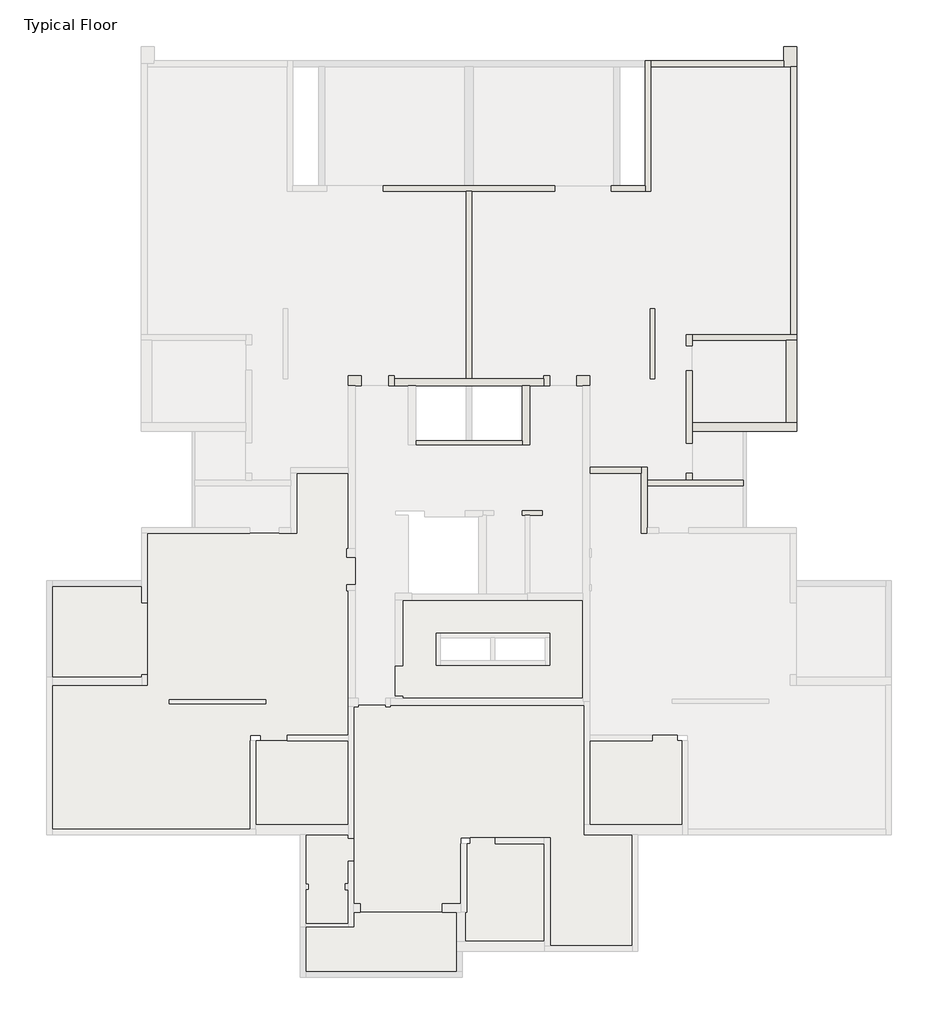
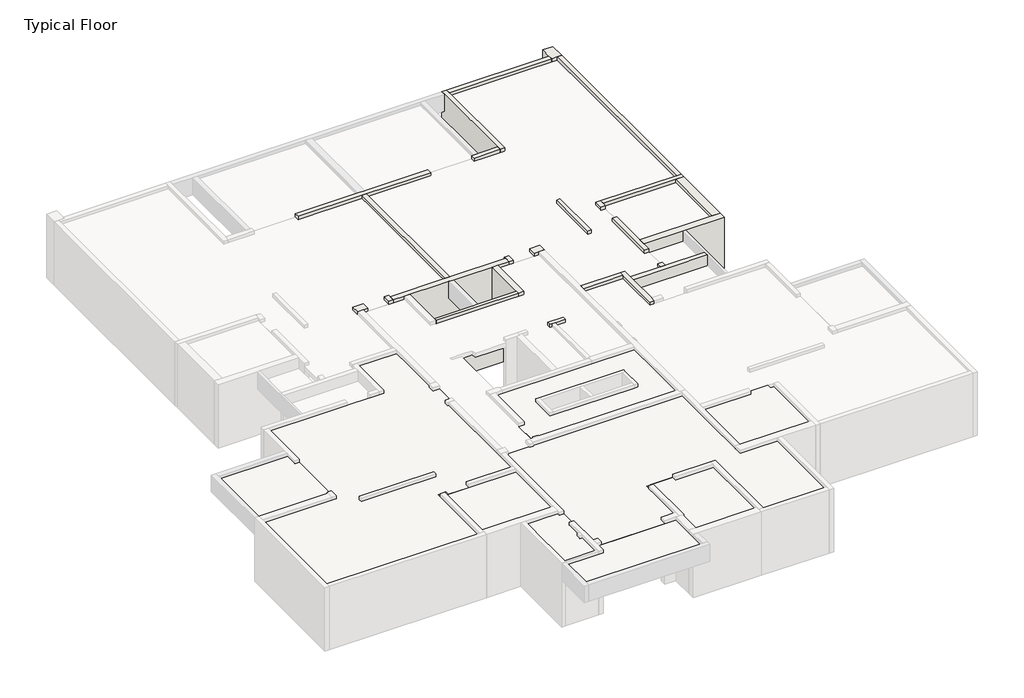
# One storey, part 3 of 4: 25 walls, 9 slabs.
"""IFC4 building model written with IfcOpenShell, lengths in millimetres."""

from ifc_helpers import new_model, si_unit, frame, origin, place, context, project, spatial, polyline, outline, extrude, faceted_brep, element, save

model = new_model("IFC4")

# Units and contexts
model_context = context("Model", 3, world=origin())
ifc_project = project(units=[si_unit("LENGTHUNIT", "METRE", prefix="MILLI")], contexts=[model_context])

# Site, building, storey
site = spatial("IfcSite", under=ifc_project)
building = spatial("IfcBuilding", under=site)
storey = spatial("IfcBuildingStorey", under=building, Name="Typical Floor", Elevation=3160.0)

# Slabs
placement = place(None, origin())
element("IfcSlab", 1, ObjectType="D=20", at=placement, inside=storey, context=model_context, shape_type="Brep", body=[
    faceted_brep([(353.6524939, -7625.251138, 2810.0), (353.6524939, -10519.1739201, 2810.0), (-2825.7294994, -10519.1739201, 2810.0), (-2825.7294994, -7625.251138, 2810.0), (-2665.7294994, -7625.251138, 2810.0), (-1746.3475061, -7625.251138, 2810.0), (353.6524939, -7625.251138, 3010.0), (-1746.3475061, -7625.251138, 3010.0), (-2665.7294994, -7625.251138, 3010.0), (-2825.7294994, -7625.251138, 3010.0), (-2825.7294994, -10519.1739201, 3010.0), (353.6524939, -10519.1739201, 3010.0)], [[[0, 1, 2, 3, 4, 5]], [[6, 7, 8, 9, 10, 11]], [[1, 0, 6, 11]], [[2, 1, 11, 10]], [[3, 2, 10, 9]], [[0, 5, 4, 3, 9, 8, 7, 6]]]),
])
element("IfcSlab", 2, ObjectType="D=20", at=placement, inside=storey, context=model_context, shape_type="SweptSolid", body=[
    extrude(outline(polyline([(353.6524939, -12752.8550877), (353.6524939, -13927.6329213), (-1104.0660909, -13927.6329213), (-1104.0660909, -12752.8550877), (-1004.0660909, -12752.8550877), (-1004.0660909, -12552.855147), (-1104.0660316, -12552.855147), (-1104.0660316, -10869.1739201), (353.6524939, -10869.1739201), (353.6524939, -10989.1739201), (553.6524939, -10989.1739201), (553.6524939, -11774.1739201), (353.6524939, -11774.1739201), (353.6524939, -12552.8550877), (253.6524939, -12552.8550877), (253.6524939, -12752.8550877), (353.6524939, -12752.8550877)])), frame((0.0, 0.0, 2810.0), z_axis=(0.0, 0.0, 1.0), x_axis=(1.0, 0.0, 0.0)), (0.0, 0.0, 1.0), 200.0),
])
element("IfcSlab", 3, ObjectType="D=20", at=placement, inside=storey, context=model_context, shape_type="Brep", body=[
    faceted_brep([(769.5270528, -13247.809147, 2810.0), (553.6524939, -13247.809147, 2810.0), (553.6524939, -11774.1739201, 2810.0), (553.6524939, -10989.1739201, 2810.0), (553.6524939, -6450.4733638, 2810.0), (703.0584279, -6450.4733638, 2810.0), (703.0584279, -6400.4733638, 2810.0), (1644.8990117, -6400.4733638, 2810.0), (1644.8990117, -6450.4733638, 2810.0), (1804.8990117, -6450.4733638, 2810.0), (1804.8990117, -6400.4733638, 2810.0), (8489.2361919, -6400.4733638, 2810.0), (8489.2361919, -10519.1739201, 2810.0), (8489.2361919, -10869.1739201, 2810.0), (10148.1730809, -10869.1739201, 2810.0), (10148.1730809, -14684.0133443, 2810.0), (7323.2436151, -14684.0133443, 2810.0), (7323.2436151, -10973.6256761, 2810.0), (7123.2436151, -10973.6256761, 2810.0), (5423.2436151, -10973.6256761, 2810.0), (4561.3412033, -10973.6256761, 2810.0), (4241.3412033, -10973.6256761, 2810.0), (4241.3412033, -11173.6256761, 2810.0), (4241.3412033, -13247.809147, 2810.0), (3603.9523756, -13247.809147, 2810.0), (3603.9523756, -13527.809147, 2810.0), (769.5270528, -13527.809147, 2810.0), (553.6524939, -13247.809147, 3010.0), (769.5270528, -13247.809147, 3010.0), (769.5270528, -13527.809147, 3010.0), (3603.9523756, -13527.809147, 3010.0), (3603.9523756, -13247.809147, 3010.0), (4241.3412033, -13247.809147, 3010.0), (4241.3412033, -11173.6256761, 3010.0), (4241.3412033, -10973.6256761, 3010.0), (4561.3412033, -10973.6256761, 3010.0), (5423.2436151, -10973.6256761, 3010.0), (7123.2436151, -10973.6256761, 3010.0), (7323.2436151, -10973.6256761, 3010.0), (7323.2436151, -14684.0133443, 3010.0), (10148.1730809, -14684.0133443, 3010.0), (10148.1730809, -10869.1739201, 3010.0), (8489.2361919, -10869.1739201, 3010.0), (8489.2361919, -10519.1739201, 3010.0), (8489.2361919, -6400.4733638, 3010.0), (1804.8990117, -6400.4733638, 3010.0), (1804.8990117, -6450.4733638, 3010.0), (1644.8990117, -6450.4733638, 3010.0), (1644.8990117, -6400.4733638, 3010.0), (703.0584279, -6400.4733638, 3010.0), (703.0584279, -6450.4733638, 3010.0), (553.6524939, -6450.4733638, 3010.0), (553.6524939, -10989.1739201, 3010.0), (553.6524939, -11774.1739201, 3010.0)], [[[0, 1, 2, 3, 4, 5, 6, 7, 8, 9, 10, 11, 12, 13, 14, 15, 16, 17, 18, 19, 20, 21, 22, 23, 24, 25, 26]], [[27, 28, 29, 30, 31, 32, 33, 34, 35, 36, 37, 38, 39, 40, 41, 42, 43, 44, 45, 46, 47, 48, 49, 50, 51, 52, 53]], [[1, 0, 28, 27]], [[4, 3, 2, 1, 27, 53, 52, 51]], [[5, 4, 51, 50]], [[6, 5, 50, 49]], [[7, 6, 49, 48]], [[8, 7, 48, 47]], [[9, 8, 47, 46]], [[10, 9, 46, 45]], [[11, 10, 45, 44]], [[11, 44, 43, 42, 13, 12]], [[14, 13, 42, 41]], [[15, 14, 41, 40]], [[16, 15, 40, 39]], [[17, 16, 39, 38]], [[17, 38, 37, 36, 35, 34, 21, 20, 19, 18]], [[21, 34, 33, 32, 23, 22]], [[24, 23, 32, 31]], [[25, 24, 31, 30]], [[26, 25, 30, 29]], [[0, 26, 29, 28]]]),
])
element("IfcSlab", 4, ObjectType="D=20", at=placement, inside=storey, context=model_context, shape_type="SweptSolid", body=[
    extrude(outline(polyline([(7123.2436151, -14534.1440447), (4393.8641143, -14534.1440447), (4393.8641143, -13527.809147), (4441.3412033, -13527.809147), (4441.3412033, -11173.6256761), (4561.3412033, -11173.6256761), (4561.3412033, -10973.6256761), (5423.2436151, -10973.6256761), (5423.2436151, -11173.6256761), (7123.2436151, -11173.6256761), (7123.2436151, -14534.1440447)])), frame((0.0, 0.0, 2810.0), z_axis=(0.0, 0.0, 1.0), x_axis=(1.0, 0.0, 0.0)), (0.0, 0.0, 1.0), 200.0),
])
element("IfcSlab", 5, ObjectType="D=20", at=placement, inside=storey, context=model_context, shape_type="SweptSolid", body=[
    extrude(outline(polyline([(11869.8374389, -7625.251138), (11869.8374389, -10519.1739201), (8689.2361919, -10519.1739201), (8689.2361919, -7625.251138), (10849.2361919, -7625.251138), (10849.2361919, -7425.251138), (11709.8374389, -7425.251138), (11709.8374389, -7625.251138), (11869.8374389, -7625.251138)])), frame((0.0, 0.0, 2810.0), z_axis=(0.0, 0.0, 1.0), x_axis=(1.0, 0.0, 0.0)), (0.0, 0.0, 1.0), 200.0),
])
element("IfcSlab", 6, ObjectType="D=20", at=placement, inside=storey, context=model_context, shape_type="Brep", body=[
    faceted_brep([(-9845.3223417, -10669.1739201, 2810.0), (-9845.3223417, -5707.6243159, 2810.0), (-6764.013165, -5707.6243159, 2810.0), (-6564.013165, -5707.6243159, 2810.0), (-6564.013165, -5351.6580536, 2810.0), (-6564.013165, -2868.5711301, 2810.0), (-6564.013165, -471.5347538, 2810.0), (-3044.013165, -471.5347538, 2810.0), (-2018.0126357, -471.5347538, 2810.0), (-1618.0126357, -471.5347538, 2810.0), (-1418.0126357, -471.5347538, 2810.0), (-1418.0126357, 1602.0583306, 2810.0), (353.0602083, 1602.0583306, 2810.0), (353.0602083, -998.8355577, 2810.0), (303.6507728, -998.8355577, 2810.0), (303.6507728, -1298.8355577, 2810.0), (603.0602083, -1298.8355577, 2810.0), (603.0602083, -2240.6761415, 2810.0), (303.6507728, -2240.6761415, 2810.0), (303.6507728, -2440.6761415, 2810.0), (353.6524939, -2440.6761415, 2810.0), (353.6524939, -6150.4733638, 2810.0), (353.6524939, -6450.4733638, 2810.0), (353.6524939, -7425.251138, 2810.0), (-1746.3475061, -7425.251138, 2810.0), (-1746.3475061, -7625.251138, 2810.0), (-2665.7294994, -7625.251138, 2810.0), (-2665.7294994, -7425.251138, 2810.0), (-3025.7294994, -7425.251138, 2810.0), (-3025.7294994, -7625.251138, 2810.0), (-3025.7294994, -10669.1739201, 2810.0), (-5822.171691, -6349.5529829, 2810.0), (-2483.2956212, -6349.5529829, 2810.0), (-2483.2956212, -6199.5529829, 2810.0), (-5822.171691, -6199.5529829, 2810.0), (-9845.3223417, -5707.6243159, 3010.0), (-9845.3223417, -10669.1739201, 3010.0), (-3025.7294994, -10669.1739201, 3010.0), (-3025.7294994, -7625.251138, 3010.0), (-3025.7294994, -7425.251138, 3010.0), (-2665.7294994, -7425.251138, 3010.0), (-2665.7294994, -7625.251138, 3010.0), (-1746.3475061, -7625.251138, 3010.0), (-1746.3475061, -7425.251138, 3010.0), (353.6524939, -7425.251138, 3010.0), (353.6524939, -6450.4733638, 3010.0), (353.6524939, -6150.4733638, 3010.0), (353.6524939, -2440.6761415, 3010.0), (303.6507728, -2440.6761415, 3010.0), (303.6507728, -2240.6761415, 3010.0), (603.0602083, -2240.6761415, 3010.0), (603.0602083, -1298.8355577, 3010.0), (303.6507728, -1298.8355577, 3010.0), (303.6507728, -998.8355577, 3010.0), (353.0602083, -998.8355577, 3010.0), (353.0602083, 1602.0583306, 3010.0), (-1418.0126357, 1602.0583306, 3010.0), (-1418.0126357, -471.5347538, 3010.0), (-1618.0126357, -471.5347538, 3010.0), (-2018.0126357, -471.5347538, 3010.0), (-3044.013165, -471.5347538, 3010.0), (-6564.013165, -471.5347538, 3010.0), (-6564.013165, -2868.5711301, 3010.0), (-6564.013165, -5351.6580536, 3010.0), (-6564.013165, -5707.6243159, 3010.0), (-6764.013165, -5707.6243159, 3010.0), (-2483.2956212, -6349.5529829, 3010.0), (-5822.171691, -6349.5529829, 3010.0), (-5822.171691, -6199.5529829, 3010.0), (-2483.2956212, -6199.5529829, 3010.0)], [[[0, 1, 2, 3, 4, 5, 6, 7, 8, 9, 10, 11, 12, 13, 14, 15, 16, 17, 18, 19, 20, 21, 22, 23, 24, 25, 26, 27, 28, 29, 30], [31, 32, 33, 34]], [[35, 36, 37, 38, 39, 40, 41, 42, 43, 44, 45, 46, 47, 48, 49, 50, 51, 52, 53, 54, 55, 56, 57, 58, 59, 60, 61, 62, 63, 64, 65], [66, 67, 68, 69]], [[1, 0, 36, 35]], [[1, 35, 65, 64, 3, 2]], [[3, 64, 63, 62, 61, 6, 5, 4]], [[6, 61, 60, 59, 58, 57, 10, 9, 8, 7]], [[11, 10, 57, 56]], [[12, 11, 56, 55]], [[13, 12, 55, 54]], [[14, 13, 54, 53]], [[15, 14, 53, 52]], [[16, 15, 52, 51]], [[17, 16, 51, 50]], [[18, 17, 50, 49]], [[19, 18, 49, 48]], [[20, 19, 48, 47]], [[20, 47, 46, 45, 44, 23, 22, 21]], [[28, 27, 40, 39]], [[28, 39, 38, 37, 30, 29]], [[0, 30, 37, 36]], [[32, 31, 67, 66]], [[34, 33, 69, 68]], [[33, 32, 66, 69]], [[31, 34, 68, 67]], [[24, 23, 44, 43]], [[25, 24, 43, 42]], [[26, 25, 42, 41]], [[27, 26, 41, 40]]]),
])
element("IfcSlab", 7, ObjectType="D=20", at=placement, inside=storey, context=model_context, shape_type="SweptSolid", body=[
    extrude(outline(polyline([(-9845.3223417, -2297.6508085), (-6764.013165, -2297.6508085), (-6764.013165, -2868.5711301), (-6564.013165, -2868.5711301), (-6564.013165, -5351.6580536), (-6764.013165, -5351.6580536), (-6764.013165, -5427.6243159), (-9845.3223417, -5427.6243159), (-9845.3223417, -2297.6508085)])), frame((0.0, 0.0, 2810.0), z_axis=(0.0, 0.0, 1.0), x_axis=(1.0, 0.0, 0.0)), (0.0, 0.0, 1.0), 200.0),
])
element("IfcSlab", 8, ObjectType="D=20", at=placement, inside=storey, context=model_context, shape_type="Brep", body=[
    faceted_brep([(353.6524939, -14027.6329213, 2810.0), (353.6524939, -14034.1739201, 2810.0), (553.6524939, -14034.1739201, 2810.0), (553.6524939, -13527.809147, 2810.0), (769.5270528, -13527.809147, 2810.0), (3603.9523756, -13527.809147, 2810.0), (4093.8641143, -13527.809147, 2810.0), (4093.8641143, -15583.8829405, 2810.0), (-1104.0660316, -15583.8829405, 2810.0), (-1104.0660316, -14027.6329213, 2810.0), (353.6524939, -14034.1739201, 3010.0), (353.6524939, -14027.6329213, 3010.0), (-1104.0660316, -14027.6329213, 3010.0), (-1104.0660316, -15583.8829405, 3010.0), (4093.8641143, -15583.8829405, 3010.0), (4093.8641143, -13527.809147, 3010.0), (3603.9523756, -13527.809147, 3010.0), (769.5270528, -13527.809147, 3010.0), (553.6524939, -13527.809147, 3010.0), (553.6524939, -14034.1739201, 3010.0)], [[[0, 1, 2, 3, 4, 5, 6, 7, 8, 9]], [[10, 11, 12, 13, 14, 15, 16, 17, 18, 19]], [[1, 0, 11, 10]], [[2, 1, 10, 19]], [[3, 2, 19, 18]], [[3, 18, 17, 16, 15, 6, 5, 4]], [[7, 6, 15, 14]], [[8, 7, 14, 13]], [[9, 8, 13, 12]], [[0, 9, 12, 11]]]),
])
element("IfcSlab", 9, ObjectType="D=20", at=placement, inside=storey, context=model_context, shape_type="Brep", body=[
    faceted_brep([(2237.3338395, -5031.1363023, 2810.0), (2237.3338395, -2776.1363023, 2810.0), (8439.2361919, -2776.1363023, 2810.0), (8439.2361919, -6150.4733638, 2810.0), (2237.3338395, -6150.4733638, 2810.0), (2237.3338395, -6084.0047389, 2810.0), (1987.3338395, -6084.0047389, 2810.0), (1987.3338395, -5031.1363023, 2810.0), (3385.5549057, -3915.4538564, 2810.0), (3385.5549057, -5009.2269053, 2810.0), (3535.5549057, -5009.2269053, 2810.0), (7154.2538596, -5009.2269053, 2810.0), (7304.2538596, -5009.2269053, 2810.0), (7304.2538596, -4065.4538564, 2810.0), (7304.2538596, -3915.4538564, 2810.0), (3535.5549057, -3915.4538564, 2810.0), (2237.3338395, -2776.1363023, 3010.0), (2237.3338395, -5031.1363023, 3010.0), (1987.3338395, -5031.1363023, 3010.0), (1987.3338395, -6084.0047389, 3010.0), (2237.3338395, -6084.0047389, 3010.0), (2237.3338395, -6150.4733638, 3010.0), (8439.2361919, -6150.4733638, 3010.0), (8439.2361919, -2776.1363023, 3010.0), (3385.5549057, -5009.2269053, 3010.0), (3385.5549057, -3915.4538564, 3010.0), (3535.5549057, -3915.4538564, 3010.0), (7304.2538596, -3915.4538564, 3010.0), (7304.2538596, -4065.4538564, 3010.0), (7304.2538596, -5009.2269053, 3010.0), (7154.2538596, -5009.2269053, 3010.0), (3535.5549057, -5009.2269053, 3010.0)], [[[0, 1, 2, 3, 4, 5, 6, 7], [8, 9, 10, 11, 12, 13, 14, 15]], [[16, 17, 18, 19, 20, 21, 22, 23], [24, 25, 26, 27, 28, 29, 30, 31]], [[1, 0, 17, 16]], [[2, 1, 16, 23]], [[3, 2, 23, 22]], [[4, 3, 22, 21]], [[5, 4, 21, 20]], [[6, 5, 20, 19]], [[7, 6, 19, 18]], [[0, 7, 18, 17]], [[29, 12, 11, 10, 9, 24, 31, 30]], [[12, 29, 28, 27, 14, 13]], [[14, 27, 26, 25, 8, 15]], [[9, 8, 25, 24]]]),
])

# Walls
element("IfcWall", 10, ObjectType="15", at=placement, inside=storey, context=model_context, shape_type="SweptSolid", body=[
    extrude(outline(polyline([(6359.8903055, 2582.4743311), (2684.2185243, 2582.4743311), (2684.2185243, 2732.4743311), (6359.8903055, 2732.4743311), (6359.8903055, 2582.4743311)])), frame((0.0, 0.0, 160.0), z_axis=(0.0, 0.0, 1.0), x_axis=(1.0, 0.0, 0.0)), (0.0, 0.0, 1.0), 3000.0),
])
element("IfcWall", 11, ObjectType="15", at=placement, inside=storey, context=model_context, shape_type="Brep", body=[
    faceted_brep([(7056.7750495, 306.3601755, 160.0), (6362.4114361, 306.3601755, 160.0), (6362.4114361, 306.3601755, 2810.0), (6362.4114361, 306.3601755, 3010.0), (6362.4114361, 306.3601755, 3160.0), (7056.7750495, 306.3601755, 3160.0), (7056.7750495, 306.3601755, 3010.0), (7056.7750495, 306.3601755, 2810.0), (7056.7750495, 156.3601755, 160.0), (7056.7750495, 156.3601755, 2810.0), (7056.7750495, 156.3601755, 3010.0), (7056.7750495, 156.3601755, 3160.0), (6609.8903055, 156.3601755, 3160.0), (6459.8903055, 156.3601755, 3160.0), (6362.4114361, 156.3601755, 3160.0), (6362.4114361, 156.3601755, 3010.0), (6362.4114361, 156.3601755, 2810.0), (6362.4114361, 156.3601755, 160.0), (6459.8903055, 156.3601755, 160.0), (6609.8903055, 156.3601755, 160.0)], [[[0, 1, 2, 3, 4, 5, 6, 7]], [[8, 9, 10, 11, 12, 13, 14, 15, 16, 17, 18, 19]], [[1, 0, 8, 19, 18, 17]], [[4, 3, 2, 1, 17, 16, 15, 14]], [[5, 4, 14, 13, 12, 11]], [[0, 7, 6, 5, 11, 10, 9, 8]]]),
])
element("IfcWall", 12, ObjectType="15", at=placement, inside=storey, context=model_context, shape_type="Brep", body=[
    faceted_brep([(10776.0680695, 7281.591066, 160.0), (10776.0680695, 4865.5631538, 160.0), (10776.0680695, 4865.5631538, 2810.0), (10776.0680695, 4865.5631538, 3010.0), (10776.0680695, 4865.5631538, 3160.0), (10776.0680695, 7281.591066, 3160.0), (10776.0680695, 7281.591066, 3010.0), (10776.0680695, 7281.591066, 2810.0), (10926.0680695, 7281.591066, 160.0), (10926.0680695, 7281.591066, 2810.0), (10926.0680695, 7281.591066, 3010.0), (10926.0680695, 7281.591066, 3160.0), (10926.0680695, 4865.5631538, 3160.0), (10926.0680695, 4865.5631538, 3010.0), (10926.0680695, 4865.5631538, 2810.0), (10926.0680695, 4865.5631538, 160.0)], [[[0, 1, 2, 3, 4, 5, 6, 7]], [[8, 9, 10, 11, 12, 13, 14, 15]], [[1, 0, 8, 15]], [[4, 3, 2, 1, 15, 14, 13, 12]], [[5, 4, 12, 11]], [[0, 7, 6, 5, 11, 10, 9, 8]]]),
])
element("IfcWall", 13, ObjectType="20", at=placement, inside=storey, context=model_context, shape_type="Brep", body=[
    faceted_brep([(10795.057825, 11324.9195447, 160.0), (10795.057825, 15624.6267847, 160.0), (10795.057825, 15824.6267847, 160.0), (10795.057825, 15824.6267847, 3160.0), (10795.057825, 15624.6267847, 3160.0), (10795.057825, 11324.9195447, 3160.0), (10795.057825, 11324.9195447, 3010.0), (10795.057825, 11324.9195447, 2810.0), (10595.057825, 11324.9195447, 160.0), (10595.057825, 11324.9195447, 3160.0), (10595.057825, 11524.9195447, 3160.0), (10595.057825, 15624.626844, 3160.0), (10595.057825, 15824.6267847, 3160.0), (10595.057825, 15824.6267847, 160.0), (10595.057825, 11524.9195447, 160.0)], [[[0, 1, 2, 3, 4, 5, 6, 7]], [[8, 9, 10, 11, 12, 13, 14]], [[2, 1, 0, 8, 14, 13]], [[5, 4, 3, 12, 11, 10, 9]], [[3, 2, 13, 12]], [[0, 7, 6, 5, 9, 8]]]),
])
element("IfcWall", 14, ObjectType="20", at=placement, inside=storey, context=model_context, shape_type="Brep", body=[
    faceted_brep([(10795.057825, 15624.6267847, 160.0), (15370.7330483, 15624.6267847, 160.0), (15370.7330483, 15624.6267847, 3160.0), (10795.057825, 15624.6267847, 3160.0), (10795.057825, 15624.6267847, 3010.0), (10795.057825, 15624.6267847, 2810.0), (10795.057825, 15824.6267847, 160.0), (10795.057825, 15824.6267847, 3160.0), (15370.7330483, 15824.6267847, 3160.0), (15370.7330483, 15824.6267847, 160.0)], [[[0, 1, 2, 3, 4, 5]], [[6, 7, 8, 9]], [[1, 0, 6, 9]], [[3, 2, 8, 7]], [[0, 5, 4, 3, 7, 6]], [[2, 1, 9, 8]]]),
])
element("IfcWall", 15, ObjectType="20", at=placement, inside=storey, context=model_context, shape_type="Brep", body=[
    faceted_brep([(15617.6160713, 15624.6267847, 160.0), (15617.6160713, 6387.8215778, 160.0), (15617.6160713, 6387.8215778, 2810.0), (15617.6160713, 6387.8215778, 3010.0), (15617.6160713, 6387.8215778, 3160.0), (15617.6160713, 15624.6267847, 3160.0), (15617.6160713, 15624.6267847, 3010.0), (15617.6160713, 15624.6267847, 2810.0), (15817.6160713, 15624.6267847, 160.0), (15817.6160713, 15624.6267847, 3160.0), (15817.6160713, 6387.8215778, 3160.0), (15817.6160713, 6387.8215778, 160.0)], [[[0, 1, 2, 3, 4, 5, 6, 7]], [[8, 9, 10, 11]], [[1, 0, 8, 11]], [[5, 4, 10, 9]], [[0, 7, 6, 5, 9, 8]], [[4, 3, 2, 1, 11, 10]]]),
])
element("IfcWall", 16, ObjectType="20", at=placement, inside=storey, context=model_context, shape_type="Brep", body=[
    faceted_brep([(15817.6160713, 6387.8215778, 160.0), (15617.6160713, 6387.8215778, 160.0), (12222.3603499, 6387.8215778, 160.0), (12222.3603499, 6387.8215778, 3160.0), (15617.6160713, 6387.8215778, 3160.0), (15817.6160713, 6387.8215778, 3160.0), (15817.6160713, 6187.8215778, 160.0), (15817.6160713, 6187.8215778, 3160.0), (15467.6160713, 6187.8215778, 3160.0), (12222.3603499, 6187.8215778, 3160.0), (12222.3603499, 6187.8215778, 160.0), (15467.6160713, 6187.8215778, 160.0)], [[[0, 1, 2, 3, 4, 5]], [[6, 7, 8, 9, 10, 11]], [[2, 1, 0, 6, 11, 10]], [[5, 4, 3, 9, 8, 7]], [[0, 5, 7, 6]], [[3, 2, 10, 9]]]),
])
element("IfcWall", 17, ObjectType="20", at=placement, inside=storey, context=model_context, shape_type="Brep", body=[
    faceted_brep([(12022.3603499, 5144.6693841, 160.0), (12022.3603499, 2644.6693841, 160.0), (12022.3603499, 2644.6693841, 2810.0), (12022.3603499, 2644.6693841, 3010.0), (12022.3603499, 2644.6693841, 3160.0), (12022.3603499, 5144.6693841, 3160.0), (12022.3603499, 5144.6693841, 3010.0), (12022.3603499, 5144.6693841, 2810.0), (12222.3603499, 5144.6693841, 160.0), (12222.3603499, 5144.6693841, 2810.0), (12222.3603499, 5144.6693841, 3010.0), (12222.3603499, 5144.6693841, 3160.0), (12222.3603499, 3348.3506111, 3160.0), (12222.3603499, 3048.3506111, 3160.0), (12222.3603499, 2644.6693841, 3160.0), (12222.3603499, 2644.6693841, 3010.0), (12222.3603499, 2644.6693841, 2810.0), (12222.3603499, 2644.6693841, 160.0), (12222.3603499, 3048.3506111, 160.0), (12222.3603499, 3348.3506111, 160.0)], [[[0, 1, 2, 3, 4, 5, 6, 7]], [[8, 9, 10, 11, 12, 13, 14, 15, 16, 17, 18, 19]], [[1, 0, 8, 19, 18, 17]], [[4, 3, 2, 1, 17, 16, 15, 14]], [[5, 4, 14, 13, 12, 11]], [[0, 7, 6, 5, 11, 10, 9, 8]]]),
])
element("IfcWall", 18, ObjectType="20", at=placement, inside=storey, context=model_context, shape_type="Brep", body=[
    faceted_brep([(4422.3514479, 11324.9195447, 160.0), (4422.3514479, 4865.5631538, 160.0), (4422.3514479, 4865.5631538, 2810.0), (4422.3514479, 4865.5631538, 3010.0), (4422.3514479, 4865.5631538, 3160.0), (4422.3514479, 11324.9195447, 3160.0), (4422.3514479, 11324.9195447, 3010.0), (4422.3514479, 11324.9195447, 2810.0), (4622.3514479, 11324.9195447, 160.0), (4622.3514479, 11324.9195447, 2810.0), (4622.3514479, 11324.9195447, 3010.0), (4622.3514479, 11324.9195447, 3160.0), (4622.3514479, 4865.5631538, 3160.0), (4622.3514479, 4865.5631538, 3010.0), (4622.3514479, 4865.5631538, 2810.0), (4622.3514479, 4865.5631538, 160.0)], [[[0, 1, 2, 3, 4, 5, 6, 7]], [[8, 9, 10, 11, 12, 13, 14, 15]], [[1, 0, 8, 15]], [[5, 4, 12, 11]], [[4, 3, 2, 1, 15, 14, 13, 12]], [[0, 7, 6, 5, 11, 10, 9, 8]]]),
])
element("IfcWall", 19, ObjectType="20", at=placement, inside=storey, context=model_context, shape_type="Brep", body=[
    faceted_brep([(1749.3507084, 4970.0149098, 160.0), (1749.3507084, 4615.5631538, 160.0), (1749.3507084, 4615.5631538, 2810.0), (1749.3507084, 4615.5631538, 3010.0), (1749.3507084, 4615.5631538, 3160.0), (1749.3507084, 4970.0149098, 3160.0), (1749.3507084, 4970.0149098, 3010.0), (1749.3507084, 4970.0149098, 2810.0), (1949.3507084, 4970.0149098, 160.0), (1949.3507084, 4970.0149098, 2810.0), (1949.3507084, 4970.0149098, 3010.0), (1949.3507084, 4970.0149098, 3160.0), (1949.3507084, 4865.5631538, 3160.0), (1949.3507084, 4615.5631538, 3160.0), (1949.3507084, 4615.5631538, 160.0), (1949.3507084, 4865.5631538, 160.0)], [[[0, 1, 2, 3, 4, 5, 6, 7]], [[8, 9, 10, 11, 12, 13, 14, 15]], [[1, 0, 8, 15, 14]], [[5, 4, 13, 12, 11]], [[0, 7, 6, 5, 11, 10, 9, 8]], [[4, 3, 2, 1, 14, 13]]]),
])
element("IfcWall", 20, ObjectType="20", at=placement, inside=storey, context=model_context, shape_type="Brep", body=[
    faceted_brep([(7104.8461452, 4970.0149098, 160.0), (7104.8461452, 4865.5631538, 160.0), (7104.8461452, 4615.5631538, 160.0), (7104.8461452, 4615.5631538, 3160.0), (7104.8461452, 4865.5631538, 3160.0), (7104.8461452, 4970.0149098, 3160.0), (7104.8461452, 4970.0149098, 3010.0), (7104.8461452, 4970.0149098, 2810.0), (7304.8461452, 4970.0149098, 160.0), (7304.8461452, 4970.0149098, 2810.0), (7304.8461452, 4970.0149098, 3010.0), (7304.8461452, 4970.0149098, 3160.0), (7304.8461452, 4615.5631538, 3160.0), (7304.8461452, 4615.5631538, 3010.0), (7304.8461452, 4615.5631538, 2810.0), (7304.8461452, 4615.5631538, 160.0)], [[[0, 1, 2, 3, 4, 5, 6, 7]], [[8, 9, 10, 11, 12, 13, 14, 15]], [[2, 1, 0, 8, 15]], [[5, 4, 3, 12, 11]], [[0, 7, 6, 5, 11, 10, 9, 8]], [[3, 2, 15, 14, 13, 12]]]),
])
element("IfcWall", 21, ObjectType="20", at=placement, inside=storey, context=model_context, shape_type="Brep", body=[
    faceted_brep([(13976.960118, 1364.6693841, 160.0), (12222.3603499, 1364.6693841, 160.0), (12022.3603499, 1364.6693841, 160.0), (10662.1205752, 1364.6693841, 160.0), (10662.1205752, 1364.6693841, 2810.0), (10662.1205752, 1364.6693841, 3010.0), (10662.1205752, 1364.6693841, 3160.0), (12022.3603499, 1364.6693841, 3160.0), (12222.3603499, 1364.6693841, 3160.0), (13976.960118, 1364.6693841, 3160.0), (13976.960118, 1364.6693841, 2660.0), (13976.960118, 1364.6693841, 2510.0), (13976.960118, 1164.6693841, 160.0), (13976.960118, 1164.6693841, 2510.0), (13976.960118, 1164.6693841, 2660.0), (13976.960118, 1164.6693841, 3160.0), (10662.1205752, 1164.6693841, 3160.0), (10662.1205752, 1164.6693841, 2660.0), (10662.1205752, 1164.6693841, 2510.0), (10662.1205752, 1164.6693841, 160.0)], [[[0, 1, 2, 3, 4, 5, 6, 7, 8, 9, 10, 11]], [[12, 13, 14, 15, 16, 17, 18, 19]], [[3, 2, 1, 0, 12, 19]], [[9, 8, 7, 6, 16, 15]], [[0, 11, 10, 9, 15, 14, 13, 12]], [[6, 5, 4, 3, 19, 18, 17, 16]]]),
])
element("IfcWall", 22, ObjectType="20", at=placement, inside=storey, context=model_context, shape_type="Brep", body=[
    faceted_brep([(10462.1205752, 1802.6523966, 160.0), (10462.1205752, 1602.6523966, 160.0), (10462.1205752, -471.5348131, 160.0), (10462.1205752, -471.5348131, 2810.0), (10462.1205752, -471.5348131, 3010.0), (10462.1205752, -471.5348131, 3160.0), (10462.1205752, 1602.6523966, 3160.0), (10462.1205752, 1802.6523966, 3160.0), (10662.1205752, 1802.6523966, 160.0), (10662.1205752, 1802.6523966, 2810.0), (10662.1205752, 1802.6523966, 3010.0), (10662.1205752, 1802.6523966, 3160.0), (10662.1205752, 1364.6693841, 3160.0), (10662.1205752, 1164.6693841, 3160.0), (10662.1205752, -271.5348131, 3160.0), (10662.1205752, -471.5348131, 3160.0), (10662.1205752, -471.5348131, 160.0), (10662.1205752, -271.5348131, 160.0), (10662.1205752, 1164.6693841, 160.0), (10662.1205752, 1364.6693841, 160.0)], [[[0, 1, 2, 3, 4, 5, 6, 7]], [[8, 9, 10, 11, 12, 13, 14, 15, 16, 17, 18, 19]], [[2, 1, 0, 8, 19, 18, 17, 16]], [[7, 6, 5, 15, 14, 13, 12, 11]], [[0, 7, 11, 10, 9, 8]], [[5, 4, 3, 2, 16, 15]]]),
])
element("IfcWall", 23, ObjectType="20", at=placement, inside=storey, context=model_context, shape_type="Brep", body=[
    faceted_brep([(8689.2361919, 1602.6523966, 160.0), (10462.1205752, 1602.6523966, 160.0), (10462.1205752, 1602.6523966, 2810.0), (10462.1205752, 1602.6523966, 3010.0), (10462.1205752, 1602.6523966, 3160.0), (8689.2361919, 1602.6523966, 3160.0), (8689.2361919, 1602.6523966, 3010.0), (8689.2361919, 1602.6523966, 2810.0), (8689.2361919, 1802.6523966, 160.0), (8689.2361919, 1802.6523966, 2810.0), (8689.2361919, 1802.6523966, 3010.0), (8689.2361919, 1802.6523966, 3160.0), (10462.1205752, 1802.6523966, 3160.0), (10462.1205752, 1802.6523966, 160.0)], [[[0, 1, 2, 3, 4, 5, 6, 7]], [[8, 9, 10, 11, 12, 13]], [[1, 0, 8, 13]], [[5, 4, 12, 11]], [[4, 3, 2, 1, 13, 12]], [[0, 7, 6, 5, 11, 10, 9, 8]]]),
])
element("IfcWall", 24, ObjectType="20", at=placement, inside=storey, context=model_context, shape_type="Brep", body=[
    faceted_brep([(10595.057825, 11524.9195447, 160.0), (9434.8198306, 11524.9195447, 160.0), (9434.8198306, 11524.9195447, 2810.0), (9434.8198306, 11524.9195447, 3010.0), (9434.8198306, 11524.9195447, 3160.0), (10595.057825, 11524.9195447, 3160.0), (10595.057825, 11324.9195447, 160.0), (10595.057825, 11324.9195447, 3160.0), (9434.8198306, 11324.9195447, 3160.0), (9434.8198306, 11324.9195447, 3010.0), (9434.8198306, 11324.9195447, 2810.0), (9434.8198306, 11324.9195447, 160.0)], [[[0, 1, 2, 3, 4, 5]], [[6, 7, 8, 9, 10, 11]], [[1, 0, 6, 11]], [[4, 3, 2, 1, 11, 10, 9, 8]], [[5, 4, 8, 7]], [[0, 5, 7, 6]]]),
])
element("IfcWall", 25, ObjectType="20", at=placement, inside=storey, context=model_context, shape_type="Brep", body=[
    faceted_brep([(7485.2622644, 11524.9195447, 160.0), (1568.9345892, 11524.9195447, 160.0), (1568.9345892, 11524.9195447, 2810.0), (1568.9345892, 11524.9195447, 3010.0), (1568.9345892, 11524.9195447, 3160.0), (7485.2622644, 11524.9195447, 3160.0), (7485.2622644, 11524.9195447, 3010.0), (7485.2622644, 11524.9195447, 2810.0), (7485.2622644, 11324.9195447, 160.0), (7485.2622644, 11324.9195447, 2810.0), (7485.2622644, 11324.9195447, 3010.0), (7485.2622644, 11324.9195447, 3160.0), (4622.3514479, 11324.9195447, 3160.0), (4422.3514479, 11324.9195447, 3160.0), (1568.9345892, 11324.9195447, 3160.0), (1568.9345892, 11324.9195447, 3010.0), (1568.9345892, 11324.9195447, 2810.0), (1568.9345892, 11324.9195447, 160.0), (4422.3514479, 11324.9195447, 160.0), (4622.3514479, 11324.9195447, 160.0)], [[[0, 1, 2, 3, 4, 5, 6, 7]], [[8, 9, 10, 11, 12, 13, 14, 15, 16, 17, 18, 19]], [[1, 0, 8, 19, 18, 17]], [[4, 3, 2, 1, 17, 16, 15, 14]], [[5, 4, 14, 13, 12, 11]], [[0, 7, 6, 5, 11, 10, 9, 8]]]),
])
element("IfcWall", 26, ObjectType="20", at=placement, inside=storey, context=model_context, shape_type="Brep", body=[
    faceted_brep([(12022.3603499, 6387.8215778, 160.0), (12022.3603499, 6007.8215778, 160.0), (12022.3603499, 6007.8215778, 2810.0), (12022.3603499, 6007.8215778, 3010.0), (12022.3603499, 6007.8215778, 3160.0), (12022.3603499, 6387.8215778, 3160.0), (12022.3603499, 6387.8215778, 3010.0), (12022.3603499, 6387.8215778, 2810.0), (12222.3603499, 6387.8215778, 160.0), (12222.3603499, 6387.8215778, 3160.0), (12222.3603499, 6187.8215778, 3160.0), (12222.3603499, 6007.8215778, 3160.0), (12222.3603499, 6007.8215778, 3010.0), (12222.3603499, 6007.8215778, 2810.0), (12222.3603499, 6007.8215778, 160.0), (12222.3603499, 6187.8215778, 160.0)], [[[0, 1, 2, 3, 4, 5, 6, 7]], [[8, 9, 10, 11, 12, 13, 14, 15]], [[1, 0, 8, 15, 14]], [[4, 3, 2, 1, 14, 13, 12, 11]], [[5, 4, 11, 10, 9]], [[0, 7, 6, 5, 9, 8]]]),
])
element("IfcWall", 27, ObjectType="20", at=placement, inside=storey, context=model_context, shape_type="Brep", body=[
    faceted_brep([(12022.3603499, 1602.6523966, 160.0), (12022.3603499, 1364.6693841, 160.0), (12022.3603499, 1364.6693841, 2810.0), (12022.3603499, 1364.6693841, 3010.0), (12022.3603499, 1364.6693841, 3160.0), (12022.3603499, 1602.6523966, 3160.0), (12022.3603499, 1602.6523966, 3010.0), (12022.3603499, 1602.6523966, 2810.0), (12222.3603499, 1602.6523966, 160.0), (12222.3603499, 1602.6523966, 2810.0), (12222.3603499, 1602.6523966, 3010.0), (12222.3603499, 1602.6523966, 3160.0), (12222.3603499, 1364.6693841, 3160.0), (12222.3603499, 1364.6693841, 160.0)], [[[0, 1, 2, 3, 4, 5, 6, 7]], [[8, 9, 10, 11, 12, 13]], [[1, 0, 8, 13]], [[5, 4, 12, 11]], [[0, 7, 6, 5, 11, 10, 9, 8]], [[4, 3, 2, 1, 13, 12]]]),
])
element("IfcWall", 28, ObjectType="25", at=placement, inside=storey, context=model_context, shape_type="Brep", body=[
    faceted_brep([(1949.3507084, 4615.5631538, 160.0), (2434.2185243, 4615.5631538, 160.0), (2684.2185243, 4615.5631538, 160.0), (6359.8903055, 4615.5631538, 160.0), (6609.8903055, 4615.5631538, 160.0), (7104.8461452, 4615.5631538, 160.0), (7104.8461452, 4615.5631538, 3160.0), (6609.8903055, 4615.5631538, 3160.0), (6359.8903055, 4615.5631538, 3160.0), (2684.2185243, 4615.5631538, 3160.0), (2434.2185243, 4615.5631538, 3160.0), (1949.3507084, 4615.5631538, 3160.0), (1949.3507084, 4865.5631538, 160.0), (1949.3507084, 4865.5631538, 2810.0), (1949.3507084, 4865.5631538, 3010.0), (1949.3507084, 4865.5631538, 3160.0), (4422.3514479, 4865.5631538, 3160.0), (4622.3514479, 4865.5631538, 3160.0), (7104.8461452, 4865.5631538, 3160.0), (7104.8461452, 4865.5631538, 3010.0), (7104.8461452, 4865.5631538, 2810.0), (7104.8461452, 4865.5631538, 160.0), (4622.3514479, 4865.5631538, 160.0), (4422.3514479, 4865.5631538, 160.0)], [[[0, 1, 2, 3, 4, 5, 6, 7, 8, 9, 10, 11]], [[12, 13, 14, 15, 16, 17, 18, 19, 20, 21, 22, 23]], [[5, 4, 3, 2, 1, 0, 12, 23, 22, 21]], [[11, 10, 9, 8, 7, 6, 18, 17, 16, 15]], [[0, 11, 15, 14, 13, 12]], [[6, 5, 21, 20, 19, 18]]]),
])
element("IfcWall", 29, ObjectType="25", at=placement, inside=storey, context=model_context, shape_type="Brep", body=[
    faceted_brep([(6609.8903055, 2582.4743311, 160.0), (6609.8903055, 4615.5631538, 160.0), (6609.8903055, 4615.5631538, 2810.0), (6609.8903055, 4615.5631538, 3010.0), (6609.8903055, 4615.5631538, 3160.0), (6609.8903055, 2582.4743311, 3160.0), (6609.8903055, 2582.4743311, 3010.0), (6609.8903055, 2582.4743311, 2810.0), (6359.8903055, 2582.4743311, 160.0), (6359.8903055, 2582.4743311, 3160.0), (6359.8903055, 2732.4743311, 3160.0), (6359.8903055, 4615.5631538, 3160.0), (6359.8903055, 4615.5631538, 160.0), (6359.8903055, 2732.4743311, 160.0)], [[[0, 1, 2, 3, 4, 5, 6, 7]], [[8, 9, 10, 11, 12, 13]], [[1, 0, 8, 13, 12]], [[5, 4, 11, 10, 9]], [[4, 3, 2, 1, 12, 11]], [[0, 7, 6, 5, 9, 8]]]),
])
element("IfcWall", 30, ObjectType="30", at=placement, inside=storey, context=model_context, shape_type="Brep", body=[
    faceted_brep([(12222.3603499, 3048.3506111, 160.0), (15817.6160713, 3048.3506111, 160.0), (15817.6160713, 3048.3506111, 3160.0), (12222.3603499, 3048.3506111, 3160.0), (12222.3603499, 3048.3506111, 2660.0), (12222.3603499, 3048.3506111, 2510.0), (12222.3603499, 3348.3506111, 160.0), (12222.3603499, 3348.3506111, 2810.0), (12222.3603499, 3348.3506111, 3010.0), (12222.3603499, 3348.3506111, 3160.0), (15467.6160713, 3348.3506111, 3160.0), (15817.6160713, 3348.3506111, 3160.0), (15817.6160713, 3348.3506111, 160.0), (15467.6160713, 3348.3506111, 160.0)], [[[0, 1, 2, 3, 4, 5]], [[6, 7, 8, 9, 10, 11, 12, 13]], [[1, 0, 6, 13, 12]], [[3, 2, 11, 10, 9]], [[0, 5, 4, 3, 9, 8, 7, 6]], [[2, 1, 12, 11]]]),
])
element("IfcWall", 31, ObjectType="35", at=placement, inside=storey, context=model_context, shape_type="Brep", body=[
    faceted_brep([(15467.6160713, 6187.8215778, 160.0), (15467.6160713, 3348.3506111, 160.0), (15467.6160713, 3348.3506111, 2810.0), (15467.6160713, 3348.3506111, 3010.0), (15467.6160713, 3348.3506111, 3160.0), (15467.6160713, 6187.8215778, 3160.0), (15817.6160713, 6187.8215778, 160.0), (15817.6160713, 6187.8215778, 3160.0), (15817.6160713, 3348.3506111, 3160.0), (15817.6160713, 3348.3506111, 160.0)], [[[0, 1, 2, 3, 4, 5]], [[6, 7, 8, 9]], [[1, 0, 6, 9]], [[5, 4, 8, 7]], [[0, 5, 7, 6]], [[4, 3, 2, 1, 9, 8]]]),
])
element("IfcWall", 32, ObjectType="45", at=placement, inside=storey, context=model_context, shape_type="Brep", body=[
    faceted_brep([(15370.7330483, 16318.9904575, 160.0), (15370.7330483, 15824.6267847, 160.0), (15370.7330483, 15624.6267847, 160.0), (15370.7330483, 15624.6267847, 3160.0), (15370.7330483, 15824.6267847, 3160.0), (15370.7330483, 16318.9904575, 3160.0), (15820.7330483, 16318.9904575, 160.0), (15820.7330483, 16318.9904575, 3160.0), (15820.7330483, 15624.6267847, 3160.0), (15820.7330483, 15624.6267847, 160.0), (15817.6160713, 15624.6267847, 160.0), (15617.6160713, 15624.6267847, 160.0), (15617.6160713, 15624.6267847, 3160.0), (15817.6160713, 15624.6267847, 3160.0)], [[[0, 1, 2, 3, 4, 5]], [[6, 7, 8, 9]], [[2, 1, 0, 6, 9, 10, 11]], [[5, 4, 3, 12, 13, 8, 7]], [[0, 5, 7, 6]], [[3, 2, 11, 10, 9, 8, 13, 12]]]),
])
element("IfcWall", 33, ObjectType="45", at=placement, inside=storey, context=model_context, shape_type="Brep", body=[
    faceted_brep([(8239.2361919, 4965.0149098, 160.0), (8239.2361919, 4613.0861241, 160.0), (8239.2361919, 4613.0861241, 2810.0), (8239.2361919, 4613.0861241, 3010.0), (8239.2361919, 4613.0861241, 3160.0), (8239.2361919, 4965.0149098, 3160.0), (8239.2361919, 4965.0149098, 3010.0), (8239.2361919, 4965.0149098, 2810.0), (8689.2361919, 4965.0149098, 160.0), (8689.2361919, 4965.0149098, 2810.0), (8689.2361919, 4965.0149098, 3010.0), (8689.2361919, 4965.0149098, 3160.0), (8689.2361919, 4613.0861241, 3160.0), (8689.2361919, 4613.0861241, 160.0), (8439.2361919, 4613.0861241, 160.0), (8439.2361919, 4613.0861241, 3160.0)], [[[0, 1, 2, 3, 4, 5, 6, 7]], [[8, 9, 10, 11, 12, 13]], [[1, 0, 8, 13, 14]], [[4, 3, 2, 1, 14, 13, 12, 15]], [[5, 4, 15, 12, 11]], [[0, 7, 6, 5, 11, 10, 9, 8]]]),
])
element("IfcWall", 34, ObjectType="45", at=placement, inside=storey, context=model_context, shape_type="Brep", body=[
    faceted_brep([(353.0602083, 4970.0149098, 160.0), (353.0602083, 4618.0861241, 160.0), (353.0602083, 4618.0861241, 3160.0), (353.0602083, 4970.0149098, 3160.0), (353.0602083, 4970.0149098, 3010.0), (353.0602083, 4970.0149098, 2810.0), (803.0602083, 4970.0149098, 160.0), (803.0602083, 4970.0149098, 2810.0), (803.0602083, 4970.0149098, 3010.0), (803.0602083, 4970.0149098, 3160.0), (803.0602083, 4618.0861241, 3160.0), (803.0602083, 4618.0861241, 3010.0), (803.0602083, 4618.0861241, 2810.0), (803.0602083, 4618.0861241, 160.0), (603.0602083, 4618.0861241, 160.0), (603.0602083, 4618.0861241, 3160.0)], [[[0, 1, 2, 3, 4, 5]], [[6, 7, 8, 9, 10, 11, 12, 13]], [[1, 0, 6, 13, 14]], [[2, 1, 14, 13, 12, 11, 10, 15]], [[3, 2, 15, 10, 9]], [[0, 5, 4, 3, 9, 8, 7, 6]]]),
])

save(model, "model.ifc")

# Revit data of these elements
# Type "D=20"
#   Function = 0
#   Layers, outside or top first: 20 cm "Concrete, Cast-in-Place - B30" (function 1)
# Type "15"
#   Layers, outside or top first: 15 cm "Concrete, Cast-in-Place - B30" (function 1)
# Type "20"
#   Layers, outside or top first: 20 cm "Concrete, Cast-in-Place - B30" (function 1)
# Type "25"
#   Layers, outside or top first: 25 cm "Concrete, Cast-in-Place - B30" (function 1)
# Type "30"
#   Layers, outside or top first: 30 cm "Concrete, Cast-in-Place - B30" (function 1)
# Type "35"
#   Layers, outside or top first: 35 cm "Concrete, Cast-in-Place - B30" (function 1)
# Type "45"
#   Layers, outside or top first: 45 cm "Concrete, Cast-in-Place - B30" (function 1)
# Element 1 (IfcSlab, "D=20")
#   Comments = ""
#   Mark = "S1"
#   SOFiSTiK_AMG_Comments = ""
#   Height Offset From Level = -15 cm
#   built-in parameter 1001954 = 1
#   SOFiSTiK_AMG_Scheduled = yes
#   SOFiSTiK_AMG_Adjusted = yes
#   Phase Created = New Construction
#   Materials on its faces: "Concrete, Cast-in-Place - B30"
# Element 2 (IfcSlab, "D=20")
#   Comments = ""
#   Mark = "S2"
#   SOFiSTiK_AMG_Comments = ""
#   Height Offset From Level = -15 cm
#   built-in parameter 1001954 = 1
#   SOFiSTiK_AMG_Scheduled = yes
#   SOFiSTiK_AMG_Adjusted = yes
#   Phase Created = New Construction
#   Materials on its faces: "Concrete, Cast-in-Place - B30"
# Element 3 (IfcSlab, "D=20")
#   Comments = ""
#   Mark = "S3"
#   SOFiSTiK_AMG_Comments = ""
#   Height Offset From Level = -15 cm
#   built-in parameter 1001954 = 1
#   SOFiSTiK_AMG_Scheduled = yes
#   SOFiSTiK_AMG_Adjusted = yes
#   Phase Created = New Construction
#   Materials on its faces: "Concrete, Cast-in-Place - B30"
# Element 4 (IfcSlab, "D=20")
#   Comments = ""
#   Mark = "S4"
#   SOFiSTiK_AMG_Comments = ""
#   Height Offset From Level = -15 cm
#   built-in parameter 1001954 = 1
#   SOFiSTiK_AMG_Scheduled = yes
#   SOFiSTiK_AMG_Adjusted = yes
#   Phase Created = New Construction
#   Materials on its faces: "Concrete, Cast-in-Place - B30"
# Element 5 (IfcSlab, "D=20")
#   Mark = "S5"
#   SOFiSTiK_AMG_Comments = ""
#   Height Offset From Level = -15 cm
#   built-in parameter 1001954 = 1
#   SOFiSTiK_AMG_Scheduled = yes
#   SOFiSTiK_AMG_Adjusted = yes
#   Phase Created = New Construction
#   Materials on its faces: "Concrete, Cast-in-Place - B30"
# Element 6 (IfcSlab, "D=20")
#   Mark = "S7"
#   SOFiSTiK_AMG_Comments = ""
#   built-in parameter 1001955 = 3.14159 (stored number, unit not read)
#   Height Offset From Level = -15 cm
#   built-in parameter 1001954 = 1
#   SOFiSTiK_AMG_Scheduled = yes
#   SOFiSTiK_AMG_Adjusted = yes
#   Phase Created = New Construction
#   Materials on its faces: "Concrete, Cast-in-Place - B30"
# Element 7 (IfcSlab, "D=20")
#   Mark = "S15"
#   SOFiSTiK_AMG_Comments = ""
#   built-in parameter 1001955 = 3.14159 (stored number, unit not read)
#   Height Offset From Level = -15 cm
#   built-in parameter 1001954 = 1
#   SOFiSTiK_AMG_Scheduled = yes
#   SOFiSTiK_AMG_Adjusted = yes
#   Phase Created = New Construction
#   Materials on its faces: "Concrete, Cast-in-Place - B30"
# Element 8 (IfcSlab, "D=20")
#   Mark = "S17"
#   SOFiSTiK_AMG_Comments = ""
#   Height Offset From Level = -15 cm
#   built-in parameter 1001954 = 1
#   SOFiSTiK_AMG_Scheduled = yes
#   SOFiSTiK_AMG_Adjusted = yes
#   Phase Created = New Construction
#   Materials on its faces: "Concrete, Cast-in-Place - B30"
# Element 9 (IfcSlab, "D=20")
#   Mark = "S18"
#   SOFiSTiK_AMG_Comments = ""
#   Height Offset From Level = -15 cm
#   built-in parameter 1001954 = 1
#   SOFiSTiK_AMG_Scheduled = yes
#   SOFiSTiK_AMG_Adjusted = yes
#   Phase Created = New Construction
#   Materials on its faces: "Concrete, Cast-in-Place - B30"
# Element 10 (IfcWall, "15")
#   Comments = ""
#   Mark = "W91"
#   SOFiSTiK_AMG_Comments = ""
#   built-in parameter 1001111 = -300 cm
#   Top Offset = 0 cm
#   Base Offset = -300 cm
#   wall height = 300 cm
#   SOFiSTiK_AMG_Scheduled = yes
#   SOFiSTiK_AMG_Adjusted = yes
#   Phase Created = New Construction
#   Base Constraint = Typical Floor
#   Top Constraint = Typical Floor
#   Materials on its faces: "Concrete, Cast-in-Place - B30"
# Element 11 (IfcWall, "15")
#   Comments = ""
#   Mark = "W94"
#   SOFiSTiK_AMG_Comments = ""
#   built-in parameter 1001111 = -300 cm
#   Top Offset = 0 cm
#   Base Offset = -300 cm
#   wall height = 300 cm
#   SOFiSTiK_AMG_Scheduled = yes
#   SOFiSTiK_AMG_Adjusted = yes
#   Phase Created = New Construction
#   Base Constraint = Typical Floor
#   Top Constraint = Typical Floor
#   Materials on its faces: "Concrete, Cast-in-Place - B30"
# Element 12 (IfcWall, "15")
#   Comments = ""
#   Mark = "W95"
#   SOFiSTiK_AMG_Comments = ""
#   built-in parameter 1001111 = -300 cm
#   Top Offset = 0 cm
#   Base Offset = -300 cm
#   wall height = 300 cm
#   SOFiSTiK_AMG_Scheduled = yes
#   SOFiSTiK_AMG_Adjusted = yes
#   Phase Created = New Construction
#   Base Constraint = Typical Floor
#   Top Constraint = Typical Floor
#   Materials on its faces: "Concrete, Cast-in-Place - B30"
# Element 13 (IfcWall, "20")
#   Comments = ""
#   Mark = "W6"
#   SOFiSTiK_AMG_Comments = ""
#   built-in parameter 1001111 = -300 cm
#   Top Offset = 0 cm
#   Base Offset = -300 cm
#   wall height = 300 cm
#   SOFiSTiK_AMG_Scheduled = yes
#   SOFiSTiK_AMG_Adjusted = yes
#   Phase Created = New Construction
#   Base Constraint = Typical Floor
#   Top Constraint = Typical Floor
#   Materials on its faces: "Concrete, Cast-in-Place - B30"
# Element 14 (IfcWall, "20")
#   Comments = ""
#   Mark = "W7"
#   SOFiSTiK_AMG_Comments = ""
#   built-in parameter 1001111 = -300 cm
#   Top Offset = 0 cm
#   Base Offset = -300 cm
#   wall height = 300 cm
#   SOFiSTiK_AMG_Scheduled = yes
#   SOFiSTiK_AMG_Adjusted = yes
#   Phase Created = New Construction
#   Base Constraint = Typical Floor
#   Top Constraint = Typical Floor
#   Materials on its faces: "Concrete, Cast-in-Place - B30"
# Element 15 (IfcWall, "20")
#   Comments = ""
#   Mark = "W8"
#   SOFiSTiK_AMG_Comments = ""
#   built-in parameter 1001111 = -300 cm
#   Top Offset = 0 cm
#   Base Offset = -300 cm
#   wall height = 300 cm
#   SOFiSTiK_AMG_Scheduled = yes
#   SOFiSTiK_AMG_Adjusted = yes
#   Phase Created = New Construction
#   Base Constraint = Typical Floor
#   Top Constraint = Typical Floor
#   Materials on its faces: "Concrete, Cast-in-Place - B30"
# Element 16 (IfcWall, "20")
#   Comments = ""
#   Mark = "W9"
#   SOFiSTiK_AMG_Comments = ""
#   built-in parameter 1001111 = -300 cm
#   Top Offset = 0 cm
#   Base Offset = -300 cm
#   wall height = 300 cm
#   SOFiSTiK_AMG_Scheduled = yes
#   SOFiSTiK_AMG_Adjusted = yes
#   Phase Created = New Construction
#   Base Constraint = Typical Floor
#   Top Constraint = Typical Floor
#   Materials on its faces: "Concrete, Cast-in-Place - B30"
# Element 17 (IfcWall, "20")
#   Comments = ""
#   Mark = "W10"
#   SOFiSTiK_AMG_Comments = ""
#   built-in parameter 1001111 = -300 cm
#   Top Offset = 0 cm
#   Base Offset = -300 cm
#   wall height = 300 cm
#   SOFiSTiK_AMG_Scheduled = yes
#   SOFiSTiK_AMG_Adjusted = yes
#   Phase Created = New Construction
#   Base Constraint = Typical Floor
#   Top Constraint = Typical Floor
#   Materials on its faces: "Concrete, Cast-in-Place - B30"
# Element 18 (IfcWall, "20")
#   Comments = ""
#   Mark = "W12"
#   SOFiSTiK_AMG_Comments = ""
#   built-in parameter 1001111 = -300 cm
#   Top Offset = 0 cm
#   Base Offset = -300 cm
#   wall height = 300 cm
#   SOFiSTiK_AMG_Scheduled = yes
#   SOFiSTiK_AMG_Adjusted = yes
#   Phase Created = New Construction
#   Base Constraint = Typical Floor
#   Top Constraint = Typical Floor
#   Materials on its faces: "Concrete, Cast-in-Place - B30"
# Element 19 (IfcWall, "20")
#   Comments = ""
#   Mark = "W13"
#   SOFiSTiK_AMG_Comments = ""
#   built-in parameter 1001111 = -300 cm
#   Top Offset = 0 cm
#   Base Offset = -300 cm
#   wall height = 300 cm
#   SOFiSTiK_AMG_Scheduled = yes
#   SOFiSTiK_AMG_Adjusted = yes
#   Phase Created = New Construction
#   Base Constraint = Typical Floor
#   Top Constraint = Typical Floor
#   Materials on its faces: "Concrete, Cast-in-Place - B30"
# Element 20 (IfcWall, "20")
#   Comments = ""
#   Mark = "W14"
#   SOFiSTiK_AMG_Comments = ""
#   built-in parameter 1001111 = -300 cm
#   Top Offset = 0 cm
#   Base Offset = -300 cm
#   wall height = 300 cm
#   SOFiSTiK_AMG_Scheduled = yes
#   SOFiSTiK_AMG_Adjusted = yes
#   Phase Created = New Construction
#   Base Constraint = Typical Floor
#   Top Constraint = Typical Floor
#   Materials on its faces: "Concrete, Cast-in-Place - B30"
# Element 21 (IfcWall, "20")
#   Comments = ""
#   Mark = "W20"
#   SOFiSTiK_AMG_Comments = ""
#   built-in parameter 1001111 = -300 cm
#   Top Offset = 0 cm
#   Base Offset = -300 cm
#   wall height = 300 cm
#   SOFiSTiK_AMG_Scheduled = yes
#   SOFiSTiK_AMG_Adjusted = yes
#   Phase Created = New Construction
#   Base Constraint = Typical Floor
#   Top Constraint = Typical Floor
#   Materials on its faces: "Concrete, Cast-in-Place - B30"
# Element 22 (IfcWall, "20")
#   Comments = ""
#   Mark = "W21"
#   SOFiSTiK_AMG_Comments = ""
#   built-in parameter 1001111 = -300 cm
#   Top Offset = 0 cm
#   Base Offset = -300 cm
#   wall height = 300 cm
#   SOFiSTiK_AMG_Scheduled = yes
#   SOFiSTiK_AMG_Adjusted = yes
#   Phase Created = New Construction
#   Base Constraint = Typical Floor
#   Top Constraint = Typical Floor
#   Materials on its faces: "Concrete, Cast-in-Place - B30"
# Element 23 (IfcWall, "20")
#   Comments = ""
#   Mark = "W43"
#   SOFiSTiK_AMG_Comments = ""
#   built-in parameter 1001111 = -300 cm
#   Top Offset = 0 cm
#   Base Offset = -300 cm
#   wall height = 300 cm
#   SOFiSTiK_AMG_Scheduled = yes
#   SOFiSTiK_AMG_Adjusted = yes
#   Phase Created = New Construction
#   Base Constraint = Typical Floor
#   Top Constraint = Typical Floor
#   Materials on its faces: "Concrete, Cast-in-Place - B30"
# Element 24 (IfcWall, "20")
#   Comments = ""
#   Mark = "W48"
#   SOFiSTiK_AMG_Comments = ""
#   built-in parameter 1001111 = -300 cm
#   Top Offset = 0 cm
#   Base Offset = -300 cm
#   wall height = 300 cm
#   SOFiSTiK_AMG_Scheduled = yes
#   SOFiSTiK_AMG_Adjusted = yes
#   Phase Created = New Construction
#   Base Constraint = Typical Floor
#   Top Constraint = Typical Floor
#   Materials on its faces: "Concrete, Cast-in-Place - B30"
# Element 25 (IfcWall, "20")
#   Comments = ""
#   Mark = "W49"
#   SOFiSTiK_AMG_Comments = ""
#   built-in parameter 1001111 = -300 cm
#   Top Offset = 0 cm
#   Base Offset = -300 cm
#   wall height = 300 cm
#   SOFiSTiK_AMG_Scheduled = yes
#   SOFiSTiK_AMG_Adjusted = yes
#   Phase Created = New Construction
#   Base Constraint = Typical Floor
#   Top Constraint = Typical Floor
#   Materials on its faces: "Concrete, Cast-in-Place - B30"
# Element 26 (IfcWall, "20")
#   Comments = ""
#   Mark = "W54"
#   SOFiSTiK_AMG_Comments = ""
#   built-in parameter 1001111 = -300 cm
#   Top Offset = 0 cm
#   Base Offset = -300 cm
#   wall height = 300 cm
#   SOFiSTiK_AMG_Scheduled = yes
#   SOFiSTiK_AMG_Adjusted = yes
#   Phase Created = New Construction
#   Base Constraint = Typical Floor
#   Top Constraint = Typical Floor
#   Materials on its faces: "Concrete, Cast-in-Place - B30"
# Element 27 (IfcWall, "20")
#   Comments = ""
#   Mark = "W55"
#   SOFiSTiK_AMG_Comments = ""
#   built-in parameter 1001111 = -300 cm
#   Top Offset = 0 cm
#   Base Offset = -300 cm
#   wall height = 300 cm
#   SOFiSTiK_AMG_Scheduled = yes
#   SOFiSTiK_AMG_Adjusted = yes
#   Phase Created = New Construction
#   Base Constraint = Typical Floor
#   Top Constraint = Typical Floor
#   Materials on its faces: "Concrete, Cast-in-Place - B30"
# Element 28 (IfcWall, "25")
#   Comments = ""
#   Mark = "W78"
#   SOFiSTiK_AMG_Comments = ""
#   built-in parameter 1001111 = -300 cm
#   Top Offset = 0 cm
#   Base Offset = -300 cm
#   wall height = 300 cm
#   SOFiSTiK_AMG_Scheduled = yes
#   SOFiSTiK_AMG_Adjusted = yes
#   Phase Created = New Construction
#   Base Constraint = Typical Floor
#   Top Constraint = Typical Floor
#   Materials on its faces: "Concrete, Cast-in-Place - B30"
# Element 29 (IfcWall, "25")
#   Comments = ""
#   Mark = "W80"
#   SOFiSTiK_AMG_Comments = ""
#   built-in parameter 1001111 = -300 cm
#   Top Offset = 0 cm
#   Base Offset = -300 cm
#   wall height = 300 cm
#   SOFiSTiK_AMG_Scheduled = yes
#   SOFiSTiK_AMG_Adjusted = yes
#   Phase Created = New Construction
#   Base Constraint = Typical Floor
#   Top Constraint = Typical Floor
#   Materials on its faces: "Concrete, Cast-in-Place - B30"
# Element 30 (IfcWall, "30")
#   Comments = ""
#   Mark = "W63"
#   SOFiSTiK_AMG_Comments = ""
#   built-in parameter 1001111 = -300 cm
#   Top Offset = 0 cm
#   Base Offset = -300 cm
#   wall height = 300 cm
#   SOFiSTiK_AMG_Scheduled = yes
#   SOFiSTiK_AMG_Adjusted = yes
#   Phase Created = New Construction
#   Base Constraint = Typical Floor
#   Top Constraint = Typical Floor
#   Materials on its faces: "Concrete, Cast-in-Place - B30"
# Element 31 (IfcWall, "35")
#   Comments = ""
#   Mark = "W70"
#   SOFiSTiK_AMG_Comments = ""
#   built-in parameter 1001111 = -300 cm
#   Top Offset = 0 cm
#   Base Offset = -300 cm
#   wall height = 300 cm
#   SOFiSTiK_AMG_Scheduled = yes
#   SOFiSTiK_AMG_Adjusted = yes
#   Phase Created = New Construction
#   Base Constraint = Typical Floor
#   Top Constraint = Typical Floor
#   Materials on its faces: "Concrete, Cast-in-Place - B30"
# Element 32 (IfcWall, "45")
#   Comments = ""
#   Mark = "W74"
#   SOFiSTiK_AMG_Comments = ""
#   built-in parameter 1001111 = -300 cm
#   Top Offset = 0 cm
#   Base Offset = -300 cm
#   wall height = 300 cm
#   SOFiSTiK_AMG_Scheduled = yes
#   SOFiSTiK_AMG_Adjusted = yes
#   Phase Created = New Construction
#   Base Constraint = Typical Floor
#   Top Constraint = Typical Floor
#   Materials on its faces: "Concrete, Cast-in-Place - B30"
# Element 33 (IfcWall, "45")
#   Comments = ""
#   Mark = "W76"
#   SOFiSTiK_AMG_Comments = ""
#   built-in parameter 1001111 = -300 cm
#   Top Offset = 0 cm
#   Base Offset = -300 cm
#   wall height = 300 cm
#   SOFiSTiK_AMG_Scheduled = yes
#   SOFiSTiK_AMG_Adjusted = yes
#   Phase Created = New Construction
#   Base Constraint = Typical Floor
#   Top Constraint = Typical Floor
#   Materials on its faces: "Concrete, Cast-in-Place - B30"
# Element 34 (IfcWall, "45")
#   Comments = ""
#   Mark = "W77"
#   SOFiSTiK_AMG_Comments = ""
#   built-in parameter 1001111 = -300 cm
#   Top Offset = 0 cm
#   Base Offset = -300 cm
#   wall height = 300 cm
#   SOFiSTiK_AMG_Scheduled = yes
#   SOFiSTiK_AMG_Adjusted = yes
#   Phase Created = New Construction
#   Base Constraint = Typical Floor
#   Top Constraint = Typical Floor
#   Materials on its faces: "Concrete, Cast-in-Place - B30"
# Materials
#   "Concrete, Cast-in-Place - B30": class "Concrete", colour RGB 192 192 192, transparency 0, Keynote = "01000", Description = "Cast-in-place concrete", Cost = 0
